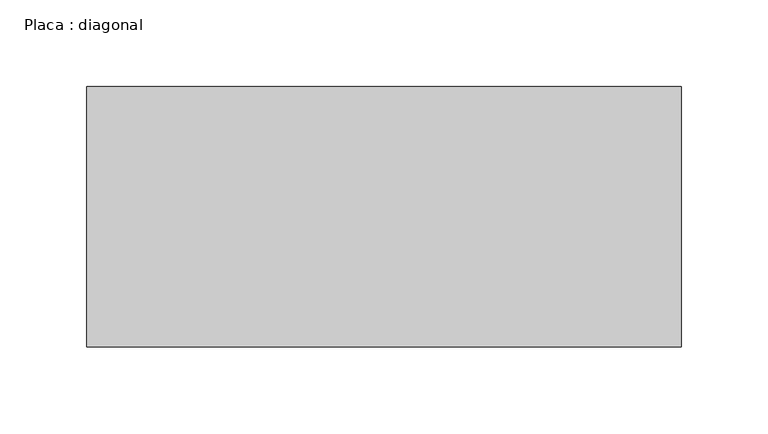
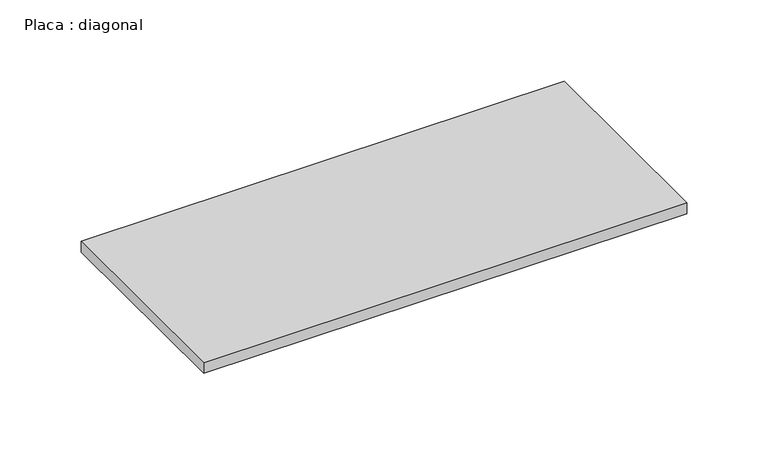
"""IFC4 building model written with IfcOpenShell, lengths in millimetres: beam geometry, Placa : diagonal."""

import ifcopenshell
import ifcopenshell.guid

model = None  # the IFC model being written
_history = None  # IfcOwnerHistory: only IFC2X3 demands one
_inside = {}  # id of a spatial element -> (the spatial element, [elements in it])
_under = {}  # id of a project, library or spatial element -> (it, [spatial elements below it])
_declared = {}  # id of a project -> (the project, [libraries it declares])
_typed = {}  # id of a type object -> (the type object, [elements of that type])
_made_of = {}  # id of a material, layer set ... -> (it, [elements and type objects made of it])


def new_model(schema):
    """Start an empty IFC model of exactly this schema.

    Asked for "IFC4X3", IfcOpenShell would pick the latest addendum, in which some entities
    have other attributes; the version numbers below select the first issue.
    IFC2X3 requires an IfcOwnerHistory on every rooted entity: one is made here for all.
    """
    global model, _history
    if schema == "IFC4X3":
        model = ifcopenshell.file(schema_version=(4, 3, 0, 0))
    else:
        model = ifcopenshell.file(schema=schema)
    _inside.clear()
    _under.clear()
    _declared.clear()
    _typed.clear()
    _made_of.clear()
    _history = None
    if model.schema == "IFC2X3":
        org = make("IfcOrganization", Name="unknown")
        user = make(
            "IfcPersonAndOrganization",
            ThePerson=make("IfcPerson", FamilyName="unknown"),
            TheOrganization=org,
        )
        app = make(
            "IfcApplication",
            ApplicationDeveloper=org,
            Version="unknown",
            ApplicationFullName="unknown",
            ApplicationIdentifier="unknown",
        )
        _history = make(
            "IfcOwnerHistory",
            OwningUser=user,
            OwningApplication=app,
            ChangeAction="ADDED",
            CreationDate=0,
        )
    return model


def make(cls, **values):
    """One entity of the class cls with the attributes given. An attribute that is None is left unset."""
    return model.create_entity(
        cls, **{name: value for name, value in values.items() if value is not None}
    )


def rooted(cls, **values):
    """An entity with a GlobalId (a new one), such as an element, a storey or a relation."""
    return make(cls, GlobalId=ifcopenshell.guid.new(), OwnerHistory=_history, **values)


def si_unit(unit_type, name, prefix=None):
    """IfcSIUnit, for example si_unit("LENGTHUNIT", "METRE", prefix="MILLI")."""
    return make("IfcSIUnit", UnitType=unit_type, Prefix=prefix, Name=name)


def assignment(units):
    """IfcUnitAssignment: the units of a project."""
    return None if units is None else make("IfcUnitAssignment", Units=units)


def point(xyz):
    """IfcCartesianPoint."""
    return None if xyz is None else make("IfcCartesianPoint", Coordinates=xyz)


def direction(xyz):
    """IfcDirection."""
    return None if xyz is None else make("IfcDirection", DirectionRatios=xyz)


def frame(location, z_axis=None, x_axis=None):
    """IfcAxis2Placement3D, a coordinate frame: its origin and axes. An axis left out is left unset."""
    return make(
        "IfcAxis2Placement3D",
        Location=point(location),
        Axis=direction(z_axis),
        RefDirection=direction(x_axis),
    )


def origin():
    """The frame at (0, 0, 0) with its axes left unset."""
    return frame((0.0, 0.0, 0.0))


def place(relative_to, where):
    """IfcLocalPlacement: puts the frame where relative to a parent placement (None: the world)."""
    return make(
        "IfcLocalPlacement", PlacementRelTo=relative_to, RelativePlacement=where
    )


def context(
    kind, dimensions, precision=None, world=None, true_north=None, identifier=None
):
    """IfcGeometricRepresentationContext, for example the 3D "Model" context."""
    return make(
        "IfcGeometricRepresentationContext",
        ContextIdentifier=identifier,
        ContextType=kind,
        CoordinateSpaceDimension=dimensions,
        Precision=precision,
        WorldCoordinateSystem=world,
        TrueNorth=true_north,
    )


def project(units=None, contexts=None):
    """IfcProject with its units and contexts."""
    return rooted(
        "IfcProject",
        Name="project",
        RepresentationContexts=contexts,
        UnitsInContext=assignment(units),
    )


def spatial(cls, under=None, at=None, **own):
    """A site, building, storey or space (cls), placed at a placement, below another one or the project."""
    s = rooted(cls, ObjectPlacement=at, **own)
    if under is not None:
        _under.setdefault(under.id(), (under, []))[1].append(s)
    return s


def polyline(points):
    """IfcPolyline through the points."""
    return make("IfcPolyline", Points=[point(p) for p in points])


def outline(outer, holes=None, kind="AREA"):
    """IfcArbitraryClosedProfileDef: a profile drawn as a closed curve; with holes, ...WithVoids."""
    if holes is None:
        return make("IfcArbitraryClosedProfileDef", ProfileType=kind, OuterCurve=outer)
    return make(
        "IfcArbitraryProfileDefWithVoids",
        ProfileType=kind,
        OuterCurve=outer,
        InnerCurves=holes,
    )


def extrude(swept, where, along, depth):
    """IfcExtrudedAreaSolid: the profile swept, set in the frame where, extruded along a direction by depth."""
    return make(
        "IfcExtrudedAreaSolid",
        SweptArea=swept,
        Position=where,
        ExtrudedDirection=direction(along),
        Depth=depth,
    )


def shape(context_of_items, identifier, shape_type, items):
    """IfcShapeRepresentation: the items that make up one representation, for example the "Body"."""
    return make(
        "IfcShapeRepresentation",
        ContextOfItems=context_of_items,
        RepresentationIdentifier=identifier,
        RepresentationType=shape_type,
        Items=items,
    )


def source(mapping_origin, context_of_items, identifier, shape_type, items):
    """IfcRepresentationMap: a shape defined once, which mapped items show again and again."""
    return make(
        "IfcRepresentationMap",
        MappingOrigin=mapping_origin,
        MappedRepresentation=shape(context_of_items, identifier, shape_type, items),
    )


def transform(
    local_origin,
    x_axis=None,
    y_axis=None,
    z_axis=None,
    scale=None,
    scale2=None,
    scale3=None,
    uniform=True,
):
    """IfcCartesianTransformationOperator3D, or its non-uniform kind. x_axis, y_axis, z_axis: its Axis1, 2, 3."""
    if uniform:
        return make(
            "IfcCartesianTransformationOperator3D",
            Axis1=direction(x_axis),
            Axis2=direction(y_axis),
            LocalOrigin=point(local_origin),
            Scale=scale,
            Axis3=direction(z_axis),
        )
    return make(
        "IfcCartesianTransformationOperator3DnonUniform",
        Axis1=direction(x_axis),
        Axis2=direction(y_axis),
        LocalOrigin=point(local_origin),
        Scale=scale,
        Axis3=direction(z_axis),
        Scale2=scale2,
        Scale3=scale3,
    )


def mapped(mapping_source, mapping_target):
    """IfcMappedItem: shows the shape of a source again, moved by a transform."""
    return make(
        "IfcMappedItem", MappingSource=mapping_source, MappingTarget=mapping_target
    )


def made_of(thing, what):
    """Note that an element or type object is made of a material, layer set ...; save() writes the relation."""
    if what is not None:
        _made_of.setdefault(what.id(), (what, []))[1].append(thing)
    return thing


def element(
    cls,
    number,
    at=None,
    inside=None,
    cuts=None,
    type_object=None,
    material=None,
    context=None,
    identifier="Body",
    shape_type=None,
    held_by="IfcProductDefinitionShape",
    body=None,
    shapes=None,
    **own,
):
    """One element of the class cls, such as IfcWall. Its Tag is "e" and its number.

    at: its placement. inside: the storey or other place that contains it. cuts: it is an
    opening in that element (IfcRelVoidsElement). A single representation is given by context,
    identifier, shape_type and body (its items); several are given by shapes. held_by: the class
    of the entity that holds the representations. save() writes the other relations.
    """
    e = rooted(cls, Tag="e%d" % number, ObjectPlacement=at, **own)
    if body is not None:
        shapes = [shape(context, identifier, shape_type, body)]
    if shapes is not None:
        e.Representation = make(held_by, Representations=shapes)
    if inside is not None:
        _inside.setdefault(inside.id(), (inside, []))[1].append(e)
    if cuts is not None:
        rooted(
            "IfcRelVoidsElement", RelatingBuildingElement=cuts, RelatedOpeningElement=e
        )
    if type_object is not None:
        _typed.setdefault(type_object.id(), (type_object, []))[1].append(e)
    return made_of(e, material)


def aggregate(whole, parts):
    """IfcRelAggregates: a whole, such as a stair, and the parts it consists of."""
    return rooted("IfcRelAggregates", RelatingObject=whole, RelatedObjects=parts)


def save(model, path):
    """Write the relations noted so far, then the file.

    IfcRelAggregates (storeys below a building ...), IfcRelContainedInSpatialStructure (elements
    in a storey), IfcRelDefinesByType, IfcRelAssociatesMaterial and IfcRelDeclares: one each for
    every whole, place, type object, material and project.
    """
    for whole, parts in _under.values():
        aggregate(whole, parts)
    for where, things in _inside.values():
        rooted(
            "IfcRelContainedInSpatialStructure",
            RelatedElements=things,
            RelatingStructure=where,
        )
    for kind, things in _typed.values():
        rooted("IfcRelDefinesByType", RelatedObjects=things, RelatingType=kind)
    for what, things in _made_of.values():
        rooted("IfcRelAssociatesMaterial", RelatedObjects=things, RelatingMaterial=what)
    for by, libraries in _declared.values():
        rooted("IfcRelDeclares", RelatingContext=by, RelatedDefinitions=libraries)
    model.write(path)


def placa_diagonal_d971223c(model_context):
    return source(origin(), model_context, "Body", "SweptSolid", [
        extrude(outline(polyline([(170.6977735, 75.0), (170.6977735, -75.0), (-171.6122365, -75.0), (-171.6122365, 75.0), (170.6977735, 75.0)])), frame((0.0, 0.0, -4.0), z_axis=(0.0, 0.0, 1.0), x_axis=(1.0, 0.0, 0.0)), (0.0, 0.0, 1.0), 8.0),
    ])


if __name__ == "__main__":
    model = new_model("IFC4")
    model_context = context("Model", 3, world=origin())
    ifc_project = project(units=[si_unit("LENGTHUNIT", "METRE", prefix="MILLI")], contexts=[model_context])
    site = spatial("IfcSite", under=ifc_project)
    building = spatial("IfcBuilding", under=site)
    placement = place(None, origin())
    placa_diagonal_shape = placa_diagonal_d971223c(model_context)
    element("IfcBeam", 1, ObjectType="Placa : diagonal", at=placement, inside=building, context=model_context, shape_type="MappedRepresentation", body=[
        mapped(placa_diagonal_shape, transform((0.0, 0.0, 0.0), x_axis=(1.0, 0.0, 0.0), y_axis=(0.0, 1.0, 0.0), z_axis=(0.0, 0.0, 1.0))),
    ])
    save(model, "model.ifc")

# Revit data of these elements
# Type "Placa : diagonal"
#   W = 0
#   Length [instance default] = 1.50 m
#   b = 0.15 m
#   d = 0.008 m
#   A = 0 m²
#   Structural Material [instance default] = Aço, 45-345
# Element 1 (IfcBeam, "Placa : diagonal")
#   Materials on its faces: "Aço, 45-345"
# Materials
#   "Aço, 45-345": class "Metal", colour RGB 247 247 247, transparency 0, Description = "Aço 345 MPa", Cost = 0
